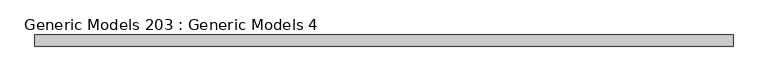
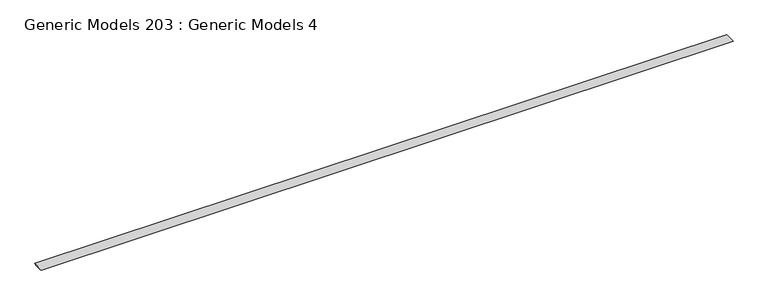
"""IFC4 building model written with IfcOpenShell, lengths in millimetres: proxy geometry, Generic Models 203 : Generic Models 4."""

from ifc_helpers import new_model, si_unit, frame, origin, place, context, project, spatial, polyline, outline, extrude, source, transform, mapped, element, save


def generic_models_203_generic_models_4_ac9a0d10(model_context):
    return source(origin(), model_context, "Body", "SweptSolid", [
        extrude(outline(polyline([(-5635.3381013, 126938.568358), (-5668.6403731, 126955.6695245), (-5469.8379675, 126959.7442042), (-5505.9091787, 126941.2211498), (-5635.3381013, 126938.568358)])), frame((-10234.5171316, 0.0, 0.0), z_axis=(1.0, 0.0, 0.0), x_axis=(0.0, 1.0, 0.0)), (0.0, 0.0, 1.0), 12431.443502),
    ])


if __name__ == "__main__":
    model = new_model("IFC4")
    model_context = context("Model", 3, world=origin())
    ifc_project = project(units=[si_unit("LENGTHUNIT", "METRE", prefix="MILLI")], contexts=[model_context])
    site = spatial("IfcSite", under=ifc_project)
    building = spatial("IfcBuilding", under=site)
    placement = place(None, origin())
    generic_models_203_generic_models_4_shape = generic_models_203_generic_models_4_ac9a0d10(model_context)
    element("IfcBuildingElementProxy", 1, Name="Generic Models 203 : Generic Models 4", ObjectType="Generic Models 203 : Generic Models 4", at=placement, inside=building, context=model_context, shape_type="MappedRepresentation", body=[
        mapped(generic_models_203_generic_models_4_shape, transform((0.0, 0.0, 0.0), x_axis=(1.0, 0.0, 0.0), y_axis=(0.0, 1.0, 0.0), z_axis=(0.0, 0.0, 1.0))),
    ])
    save(model, "model.ifc")

# Revit data of these elements
# Element 1 (IfcBuildingElementProxy, "Generic Models 203 : Generic Models 4")
#   Materials on its faces: "_7/8\" SMOOTH TROWEL EXTERIOR STUCCO (COLOR PER OWNER) @ 2% SLOPE"
# Materials
#   "_7/8\" SMOOTH TROWEL EXTERIOR STUCCO (COLOR PER OWNER) @ 2% SLOPE": class "Generic", colour RGB 233 233 233, transparency 0, Cost = 0
